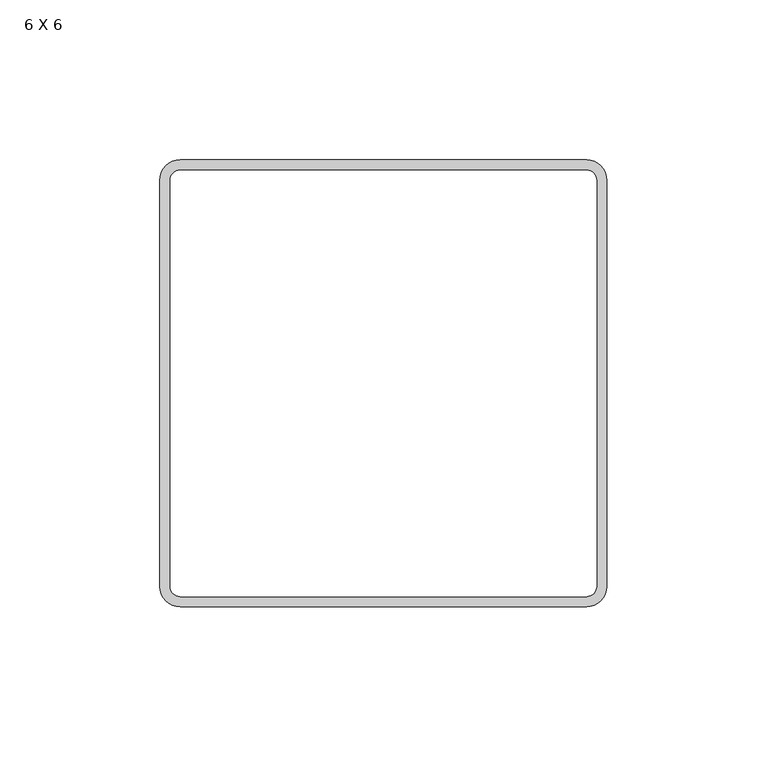
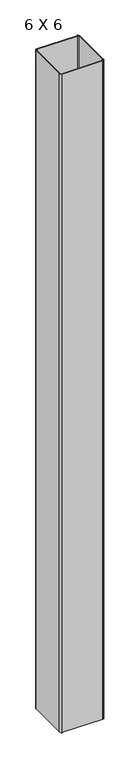
"""IFC4 building model written with IfcOpenShell, lengths in millimetres: column geometry, Structural_Column-Trex-Deck_Support_Post : 6 X 6."""

from ifc_helpers import new_model, si_unit, point, frame, frame_2d, origin, place, context, project, spatial, polyline, circle_curve, trimmed, segment, composite_curve, outline, extrude, source, transform, mapped, element, save


def column_6_x_6_a355857d(model_context):
    return source(origin(), model_context, "Body", "SweptSolid", [
        extrude(outline(composite_curve([segment(polyline([(-63.5, 69.85), (63.5, 69.85)]), True, "CONTINUOUS"), segment(trimmed(circle_curve(frame_2d((63.5, 63.5)), 6.35), [point((63.5, 69.85))], [point((69.85, 63.5))], False, "CARTESIAN"), True, "CONTINUOUS"), segment(polyline([(69.85, 63.5), (69.85, -63.5)]), True, "CONTINUOUS"), segment(trimmed(circle_curve(frame_2d((63.5, -63.5)), 6.35), [point((69.85, -63.5))], [point((63.5, -69.85))], False, "CARTESIAN"), True, "CONTINUOUS"), segment(polyline([(63.5, -69.85), (-63.5, -69.85)]), True, "CONTINUOUS"), segment(trimmed(circle_curve(frame_2d((-63.5, -63.5)), 6.35), [point((-63.5, -69.85))], [point((-69.85, -63.5))], False, "CARTESIAN"), True, "CONTINUOUS"), segment(polyline([(-69.85, -63.5), (-69.85, 63.5)]), True, "CONTINUOUS"), segment(trimmed(circle_curve(frame_2d((-63.5, 63.5)), 6.35), [point((-69.85, 63.5))], [point((-63.5, 69.85))], False, "CARTESIAN"), True, "CONTINUOUS")], self_intersect=False), holes=[composite_curve([segment(trimmed(circle_curve(frame_2d((-63.5, 63.5)), 3.175), [point((-63.5, 66.675))], [point((-66.675, 63.5))], True, "CARTESIAN"), True, "CONTINUOUS"), segment(polyline([(-66.675, 63.5), (-66.675, -63.5)]), True, "CONTINUOUS"), segment(trimmed(circle_curve(frame_2d((-63.5, -63.5)), 3.175), [point((-66.675, -63.5))], [point((-63.5, -66.675))], True, "CARTESIAN"), True, "CONTINUOUS"), segment(polyline([(-63.5, -66.675), (63.5, -66.675)]), True, "CONTINUOUS"), segment(trimmed(circle_curve(frame_2d((63.5, -63.5)), 3.175), [point((63.5, -66.675))], [point((66.675, -63.5))], True, "CARTESIAN"), True, "CONTINUOUS"), segment(polyline([(66.675, -63.5), (66.675, 63.5)]), True, "CONTINUOUS"), segment(trimmed(circle_curve(frame_2d((63.5, 63.5)), 3.175), [point((66.675, 63.5))], [point((63.5, 66.675))], True, "CARTESIAN"), True, "CONTINUOUS"), segment(polyline([(63.5, 66.675), (-63.5, 66.675)]), True, "CONTINUOUS")], self_intersect=False)]), frame((0.0, 0.0, 2784.475), z_axis=(0.0, 0.0, 1.0), x_axis=(1.0, 0.0, 0.0)), (0.0, 0.0, 1.0), 2200.275),
    ])


if __name__ == "__main__":
    model = new_model("IFC4")
    model_context = context("Model", 3, world=origin())
    ifc_project = project(units=[si_unit("LENGTHUNIT", "METRE", prefix="MILLI")], contexts=[model_context])
    site = spatial("IfcSite", under=ifc_project)
    building = spatial("IfcBuilding", under=site)
    placement = place(None, origin())
    column_6_x_6_shape = column_6_x_6_a355857d(model_context)
    element("IfcColumn", 1, ObjectType="Structural_Column-Trex-Deck_Support_Post : 6 X 6", at=placement, inside=building, context=model_context, shape_type="MappedRepresentation", body=[
        mapped(column_6_x_6_shape, transform((0.0, 0.0, 0.0), x_axis=(1.0, 0.0, 0.0), y_axis=(0.0, 1.0, 0.0), z_axis=(0.0, 0.0, 1.0))),
    ])
    save(model, "model.ifc")

# Revit data of these elements
# Type "Structural_Column-Trex-Deck_Support_Post : 6 X 6"
#   URL = "www.trex.com"
#   Product Page URL = "http://www.trex.com/products/deck-framing-drainage/elevations/"
#   Product Name = "Trex Elevations® Support Post"
#   Product Documentation Link = "http://www.trex.com/trex/groups/content/@mktgtechsvc/documents/document/trexmd_010019.pdf"
#   Model = "Support Post"
#   Material = ""
#   Manufacturer = "Trex®"
#   Description = "Steel Deck Framing"
#   Width = 0' - 5 1/2"
#   Thickness = 0' - 0 1/8"
#   Depth = 0' - 5 1/2"
#   Detail Component = yes
#   Structural Material [instance default] = Metal Joists - Trex - Elevations® Steel Deck Framing - 2x8
# Element 1 (IfcColumn, "Structural_Column-Trex-Deck_Support_Post : 6 X 6")
#   Structural Material = ALL 5.5"X5.5" GLULAM COLUMNS - ARCHITECTURAL APPEARANCE - FINISH ALL 4 SIDES - STAIN T.B.D.
#   Materials on its faces: "ALL 5.5\"X5.5\" GLULAM COLUMNS - ARCHITECTURAL APPEARANCE - FINISH ALL 4 SIDES - STAIN T.B.D."
# Materials
#   "Metal Joists - Trex - Elevations® Steel Deck Framing - 2x8": class "Wood", colour RGB 114 102 88, transparency 0, Keynote = "05 42 16", Model = "Trex Elevations® Steel Deck Framing", Manufacturer = "Trex", URL = "http://www.trex.com/", Description = "2x8 Trex Elevations® Steel Deck Framing", Cost = 0
#   "ALL 5.5\"X5.5\" GLULAM COLUMNS - ARCHITECTURAL APPEARANCE - FINISH ALL 4 SIDES - STAIN T.B.D.": class "Wood", colour RGB 234 198 147, transparency 0, Description = "Pinus Echinata", Cost = 0
